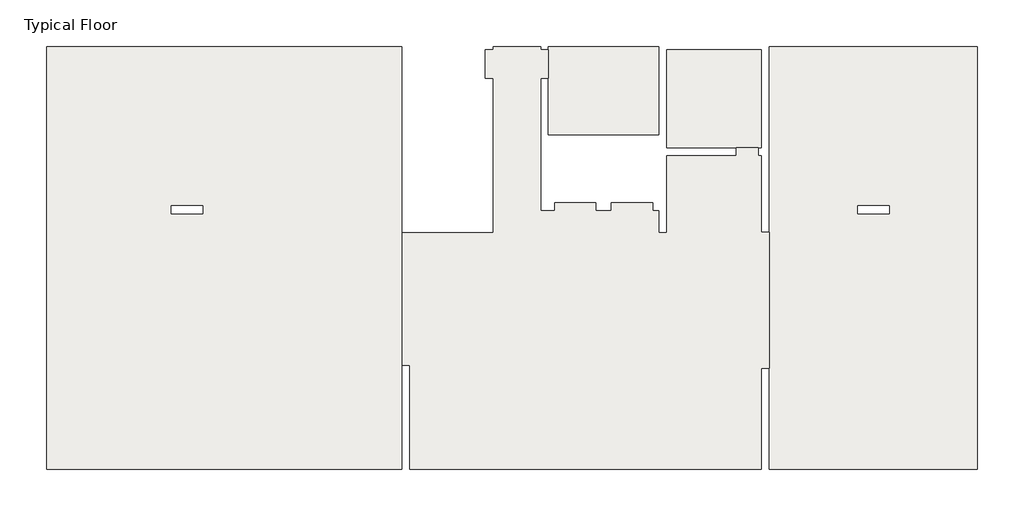
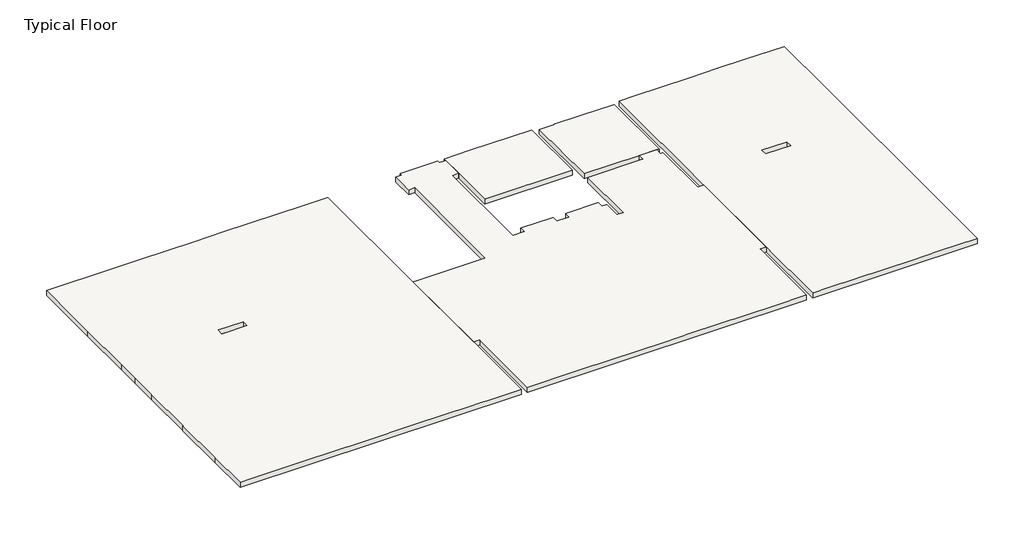
# One storey: 5 slabs.
"""IFC4 building model written with IfcOpenShell, lengths in millimetres."""

from ifc_helpers import new_model, si_unit, origin, place, context, project, spatial, faceted_brep, element, save

model = new_model("IFC4")

# Units and contexts
model_context = context("Model", 3, world=origin())
ifc_project = project(units=[si_unit("LENGTHUNIT", "METRE", prefix="MILLI")], contexts=[model_context])

# Site, building, storey
site = spatial("IfcSite", under=ifc_project)
building = spatial("IfcBuilding", under=site)
storey = spatial("IfcBuildingStorey", under=building, Name="Typical Floor", Elevation=3500.0)

# Slabs
placement = place(None, origin())
element("IfcSlab", 1, ObjectType="21", at=placement, inside=storey, context=model_context, shape_type="Brep", body=[
    faceted_brep([(67.1459865, 8440.4665211, 3290.0), (67.1459865, 2544.8683269, 3290.0), (67.1459865, -1658.0097769, 3290.0), (67.1459865, -4954.849506, 3290.0), (-11182.5718465, -4954.849506, 3290.0), (-11182.5718465, -3207.1068424, 3290.0), (-11187.5718465, -3207.1068424, 3290.0), (-11187.5718465, -1006.2039078, 3290.0), (-11182.5718465, -1006.2039078, 3290.0), (-11182.5718465, 1194.6990267, 3290.0), (-11187.5718465, 1194.6990267, 3290.0), (-11187.5718465, 2290.9179883, 3290.0), (-11182.5718465, 2290.9179883, 3290.0), (-11182.5718465, 3268.626792, 3290.0), (-11187.5718465, 3268.626792, 3290.0), (-11187.5718465, 5592.2723901, 3290.0), (-11182.5718465, 5592.2723901, 3290.0), (-11182.5718465, 8440.4665211, 3290.0), (-6230.8224108, 3391.6516226, 3290.0), (-7230.8224108, 3391.6516226, 3290.0), (-7230.8224108, 3141.6516226, 3290.0), (-6230.8224108, 3141.6516226, 3290.0), (67.1459865, -4954.849506, 3500.0), (67.1459865, -1658.0097769, 3500.0), (67.1459865, 2544.8683269, 3500.0), (67.1459865, 8440.4665211, 3500.0), (-830.1452099, 8440.4665211, 3500.0), (-1930.5966772, 8440.4665211, 3500.0), (-4131.4996117, 8440.4665211, 3500.0), (-5232.8540135, 8440.4665211, 3500.0), (-7432.8540135, 8440.4665211, 3500.0), (-8529.0729751, 8440.4665211, 3500.0), (-11182.5718465, 8440.4665211, 3500.0), (-11182.5718465, 5592.2723901, 3500.0), (-11187.5718465, 5592.2723901, 3500.0), (-11187.5718465, 3268.626792, 3500.0), (-11182.5718465, 3268.626792, 3500.0), (-11182.5718465, 2290.9179883, 3500.0), (-11187.5718465, 2290.9179883, 3500.0), (-11187.5718465, 1194.6990267, 3500.0), (-11182.5718465, 1194.6990267, 3500.0), (-11182.5718465, -1006.2039078, 3500.0), (-11187.5718465, -1006.2039078, 3500.0), (-11187.5718465, -3207.1068424, 3500.0), (-11182.5718465, -3207.1068424, 3500.0), (-11182.5718465, -4954.849506, 3500.0), (-8529.0729751, -4954.849506, 3500.0), (-7432.8540135, -4954.849506, 3500.0), (-6332.4025462, -4954.849506, 3500.0), (-4131.4996117, -4954.849506, 3500.0), (-1930.5966772, -4954.849506, 3500.0), (-830.1452099, -4954.849506, 3500.0), (-7230.8224108, 3391.6516226, 3500.0), (-6230.8224108, 3391.6516226, 3500.0), (-6230.8224108, 3141.6516226, 3500.0), (-7230.8224108, 3141.6516226, 3500.0)], [[[0, 1, 2, 3, 4, 5, 6, 7, 8, 9, 10, 11, 12, 13, 14, 15, 16, 17], [18, 19, 20, 21]], [[22, 23, 24, 25, 26, 27, 28, 29, 30, 31, 32, 33, 34, 35, 36, 37, 38, 39, 40, 41, 42, 43, 44, 45, 46, 47, 48, 49, 50, 51], [52, 53, 54, 55]], [[3, 2, 1, 0, 25, 24, 23, 22]], [[3, 22, 51, 50, 49, 48, 47, 46, 45, 4]], [[6, 43, 42, 7]], [[10, 39, 38, 11]], [[14, 35, 34, 15]], [[25, 0, 17, 32, 31, 30, 29, 28, 27, 26]], [[18, 53, 52, 19]], [[53, 18, 21, 54]], [[54, 21, 20, 55]], [[55, 20, 19, 52]], [[44, 5, 4, 45]], [[5, 44, 43, 6]], [[8, 41, 40, 9]], [[9, 40, 39, 10]], [[41, 8, 7, 42]], [[12, 37, 36, 13]], [[13, 36, 35, 14]], [[37, 12, 11, 38]], [[16, 33, 32, 17]], [[33, 16, 15, 34]]]),
])
element("IfcSlab", 2, ObjectType="21", at=placement, inside=storey, context=model_context, shape_type="Brep", body=[
    faceted_brep([(2966.4123522, 2544.8683269, 3290.0), (2966.4123522, 7441.8773563, 3290.0), (2716.4123522, 7441.8773563, 3290.0), (2716.4123522, 8343.4010583, 3290.0), (2966.4123522, 8343.4010583, 3290.0), (2966.4123522, 8440.4665211, 3290.0), (4468.6696885, 8440.4665211, 3290.0), (4468.6696885, 8343.4010583, 3290.0), (4718.6696885, 8343.4010583, 3290.0), (4718.6696885, 7441.8773563, 3290.0), (4468.9518556, 7441.8773563, 3290.0), (4468.9518556, 3493.2317581, 3290.0), (4468.9518556, 3243.2317581, 3290.0), (4926.0624651, 3243.2317581, 3290.0), (4926.0624651, 3493.2317581, 3290.0), (6216.9766863, 3493.2317581, 3290.0), (6216.9766863, 3243.2317581, 3290.0), (6716.4123522, 3243.2317581, 3290.0), (6716.4123522, 3493.2317581, 3290.0), (8020.0240903, 3493.2317581, 3290.0), (8020.0240903, 3243.2317581, 3290.0), (8218.6696885, 3243.2317581, 3290.0), (8218.6696885, 2544.8683269, 3290.0), (8468.6696885, 2544.8683269, 3290.0), (8468.6696885, 4990.9744217, 3290.0), (10669.5726231, 4990.9744217, 3290.0), (10669.5726231, 5240.9744217, 3290.0), (11372.1685599, 5240.9744217, 3290.0), (11372.1685599, 4991.2565888, 3290.0), (11469.2340226, 4991.2565888, 3290.0), (11469.2340226, 2566.0308552, 3290.0), (11719.2340226, 2566.0308552, 3290.0), (11719.2340226, -1755.3574067, 3290.0), (11469.2340226, -1755.3574067, 3290.0), (11469.2340226, -4954.849506, 3290.0), (317.1459865, -4954.849506, 3290.0), (317.1459865, -1658.0097769, 3290.0), (67.1459865, -1658.0097769, 3290.0), (67.1459865, 2544.8683269, 3290.0), (317.1459865, 2544.8683269, 3290.0), (2716.4123522, 2544.8683269, 3290.0), (2966.4123522, 7441.8773563, 3500.0), (2966.4123522, 2544.8683269, 3500.0), (2716.4123522, 2544.8683269, 3500.0), (317.1459865, 2544.8683269, 3500.0), (67.1459865, 2544.8683269, 3500.0), (67.1459865, -1658.0097769, 3500.0), (317.1459865, -1658.0097769, 3500.0), (317.1459865, -4954.849506, 3500.0), (2466.9766863, -4954.849506, 3500.0), (5768.3310881, -4954.849506, 3500.0), (6868.7825554, -4954.849506, 3500.0), (9069.6854899, -4954.849506, 3500.0), (10165.9044515, -4954.849506, 3500.0), (11469.2340226, -4954.849506, 3500.0), (11469.2340226, -1755.3574067, 3500.0), (11719.2340226, -1755.3574067, 3500.0), (11719.2340226, 2566.0308552, 3500.0), (11469.2340226, 2566.0308552, 3500.0), (11469.2340226, 4991.2565888, 3500.0), (11372.1685599, 4991.2565888, 3500.0), (11372.1685599, 5240.9744217, 3500.0), (10669.5726231, 5240.9744217, 3500.0), (10669.5726231, 4990.9744217, 3500.0), (8468.6696885, 4990.9744217, 3500.0), (8468.6696885, 2544.8683269, 3500.0), (8218.6696885, 2544.8683269, 3500.0), (8218.6696885, 3243.2317581, 3500.0), (8020.0240903, 3243.2317581, 3500.0), (8020.0240903, 3493.2317581, 3500.0), (6716.4123522, 3493.2317581, 3500.0), (6716.4123522, 3243.2317581, 3500.0), (6216.9766863, 3243.2317581, 3500.0), (6216.9766863, 3493.2317581, 3500.0), (4926.0624651, 3493.2317581, 3500.0), (4926.0624651, 3243.2317581, 3500.0), (4468.9518556, 3243.2317581, 3500.0), (4468.9518556, 3493.2317581, 3500.0), (4468.9518556, 7441.8773563, 3500.0), (4718.6696885, 7441.8773563, 3500.0), (4718.6696885, 8343.4010583, 3500.0), (4468.6696885, 8343.4010583, 3500.0), (4468.6696885, 8440.4665211, 3500.0), (2966.4123522, 8440.4665211, 3500.0), (2966.4123522, 8343.4010583, 3500.0), (2716.4123522, 8343.4010583, 3500.0), (2716.4123522, 7441.8773563, 3500.0)], [[[0, 1, 2, 3, 4, 5, 6, 7, 8, 9, 10, 11, 12, 13, 14, 15, 16, 17, 18, 19, 20, 21, 22, 23, 24, 25, 26, 27, 28, 29, 30, 31, 32, 33, 34, 35, 36, 37, 38, 39, 40]], [[41, 42, 43, 44, 45, 46, 47, 48, 49, 50, 51, 52, 53, 54, 55, 56, 57, 58, 59, 60, 61, 62, 63, 64, 65, 66, 67, 68, 69, 70, 71, 72, 73, 74, 75, 76, 77, 78, 79, 80, 81, 82, 83, 84, 85, 86]], [[1, 0, 42, 41]], [[6, 5, 83, 82]], [[10, 78, 77, 76, 12, 11]], [[22, 21, 67, 66]], [[23, 22, 66, 65]], [[24, 23, 65, 64]], [[30, 29, 59, 58]], [[31, 30, 58, 57]], [[32, 31, 57, 56]], [[33, 32, 56, 55]], [[34, 33, 55, 54]], [[35, 34, 54, 53, 52, 51, 50, 49, 48]], [[36, 35, 48, 47]], [[37, 36, 47, 46]], [[38, 37, 46, 45]], [[38, 45, 44, 43, 42, 0, 40, 39]], [[2, 1, 41, 86]], [[3, 2, 86, 85]], [[4, 3, 85, 84]], [[5, 4, 84, 83]], [[7, 6, 82, 81]], [[8, 7, 81, 80]], [[9, 8, 80, 79]], [[10, 9, 79, 78]], [[13, 12, 76, 75]], [[14, 13, 75, 74]], [[15, 14, 74, 73]], [[16, 15, 73, 72]], [[17, 16, 72, 71]], [[18, 17, 71, 70]], [[19, 18, 70, 69]], [[20, 19, 69, 68]], [[21, 20, 68, 67]], [[25, 24, 64, 63]], [[26, 25, 63, 62]], [[27, 26, 62, 61]], [[28, 27, 61, 60]], [[29, 28, 60, 59]]]),
])
element("IfcSlab", 3, ObjectType="21", at=placement, inside=storey, context=model_context, shape_type="Brep", body=[
    faceted_brep([(18317.4281535, -4954.849506, 3290.0), (11719.2340226, -4954.849506, 3290.0), (11719.2340226, -1755.3574067, 3290.0), (11719.2340226, 2566.0308552, 3290.0), (11719.2340226, 8440.7486881, 3290.0), (14567.7103206, 8440.7486881, 3290.0), (14567.7103206, 8440.4665211, 3290.0), (15668.1617879, 8440.4665211, 3290.0), (15668.1617879, 8440.7486881, 3290.0), (16768.6132551, 8440.7486881, 3290.0), (16768.6132551, 8440.4665211, 3290.0), (18317.4281535, 8440.4665211, 3290.0), (15515.7915847, 3391.6516226, 3290.0), (14515.7915847, 3391.6516226, 3290.0), (14515.7915847, 3141.6516226, 3290.0), (15515.7915847, 3141.6516226, 3290.0), (11719.2340226, -4954.849506, 3500.0), (12366.8073861, -4954.849506, 3500.0), (13467.2588533, -4954.849506, 3500.0), (15668.1617879, -4954.849506, 3500.0), (16768.6132551, -4954.849506, 3500.0), (18317.4281535, -4954.849506, 3500.0), (18317.4281535, -3207.1068424, 3500.0), (18317.4281535, -2106.6553751, 3500.0), (18317.4281535, 1194.6990267, 3500.0), (18317.4281535, 2290.9179883, 3500.0), (18317.4281535, 4491.8209229, 3500.0), (18317.4281535, 5600.7374014, 3500.0), (18317.4281535, 8440.4665211, 3500.0), (16768.6132551, 8440.4665211, 3500.0), (16768.6132551, 8440.7486881, 3500.0), (15668.1617879, 8440.7486881, 3500.0), (15668.1617879, 8440.4665211, 3500.0), (14567.7103206, 8440.4665211, 3500.0), (14567.7103206, 8440.7486881, 3500.0), (12366.8073861, 8440.7486881, 3500.0), (11719.2340226, 8440.7486881, 3500.0), (11719.2340226, 2566.0308552, 3500.0), (11719.2340226, -1755.3574067, 3500.0), (14515.7915847, 3391.6516226, 3500.0), (15515.7915847, 3391.6516226, 3500.0), (15515.7915847, 3141.6516226, 3500.0), (14515.7915847, 3141.6516226, 3500.0)], [[[0, 1, 2, 3, 4, 5, 6, 7, 8, 9, 10, 11], [12, 13, 14, 15]], [[16, 17, 18, 19, 20, 21, 22, 23, 24, 25, 26, 27, 28, 29, 30, 31, 32, 33, 34, 35, 36, 37, 38], [39, 40, 41, 42]], [[21, 0, 11, 28, 27, 26, 25, 24, 23, 22]], [[1, 0, 21, 20, 19, 18, 17, 16]], [[4, 3, 2, 1, 16, 38, 37, 36]], [[8, 31, 30, 9]], [[4, 36, 35, 34, 5]], [[12, 40, 39, 13]], [[40, 12, 15, 41]], [[41, 15, 14, 42]], [[42, 14, 13, 39]], [[6, 33, 32, 7]], [[7, 32, 31, 8]], [[33, 6, 5, 34]], [[10, 29, 28, 11]], [[29, 10, 9, 30]]]),
])
element("IfcSlab", 4, ObjectType="21", at=placement, inside=storey, context=model_context, shape_type="Brep", body=[
    faceted_brep([(8218.6696885, 5643.0624579, 3290.0), (4718.9518556, 5643.0624579, 3290.0), (4718.9518556, 7441.8773563, 3290.0), (4718.6696885, 7441.8773563, 3290.0), (4718.6696885, 8343.4010583, 3290.0), (4718.6696885, 8445.4665211, 3290.0), (5768.3310881, 8445.4665211, 3290.0), (5768.3310881, 8440.4665211, 3290.0), (8218.6696885, 8440.4665211, 3290.0), (4718.9518556, 5643.0624579, 3500.0), (8218.6696885, 5643.0624579, 3500.0), (8218.6696885, 8440.4665211, 3500.0), (5768.3310881, 8440.4665211, 3500.0), (5768.3310881, 8445.4665211, 3500.0), (4718.6696885, 8445.4665211, 3500.0), (4718.6696885, 8343.4010583, 3500.0), (4718.6696885, 7441.8773563, 3500.0), (4718.9518556, 7441.8773563, 3500.0)], [[[0, 1, 2, 3, 4, 5, 6, 7, 8]], [[9, 10, 11, 12, 13, 14, 15, 16, 17]], [[14, 5, 4, 3, 16, 15]], [[5, 14, 13, 6]], [[10, 0, 8, 11]], [[0, 10, 9, 1]], [[17, 2, 1, 9]], [[2, 17, 16, 3]], [[7, 12, 11, 8]], [[12, 7, 6, 13]]]),
])
element("IfcSlab", 5, ObjectType="21", at=placement, inside=storey, context=model_context, shape_type="Brep", body=[
    faceted_brep([(11469.2340226, 5241.2565888, 3290.0), (11372.1685599, 5241.2565888, 3290.0), (11372.1685599, 5240.9744217, 3290.0), (10669.5726231, 5240.9744217, 3290.0), (8468.6696885, 5240.9744217, 3290.0), (8468.6696885, 8340.4665211, 3290.0), (9069.6854899, 8340.4665211, 3290.0), (9069.6854899, 8345.4665211, 3290.0), (10165.9044515, 8345.4665211, 3290.0), (10165.9044515, 8340.4665211, 3290.0), (11469.2340226, 8340.4665211, 3290.0), (11372.1685599, 5241.2565888, 3500.0), (11469.2340226, 5241.2565888, 3500.0), (11469.2340226, 8340.4665211, 3500.0), (10165.9044515, 8340.4665211, 3500.0), (10165.9044515, 8345.4665211, 3500.0), (9069.6854899, 8345.4665211, 3500.0), (9069.6854899, 8340.4665211, 3500.0), (8468.6696885, 8340.4665211, 3500.0), (8468.6696885, 5240.9744217, 3500.0), (10669.5726231, 5240.9744217, 3500.0), (11372.1685599, 5240.9744217, 3500.0)], [[[0, 1, 2, 3, 4, 5, 6, 7, 8, 9, 10]], [[11, 12, 13, 14, 15, 16, 17, 18, 19, 20, 21]], [[12, 0, 10, 13]], [[19, 4, 3, 2, 21, 20]], [[4, 19, 18, 5]], [[7, 16, 15, 8]], [[11, 1, 0, 12]], [[1, 11, 21, 2]], [[17, 6, 5, 18]], [[6, 17, 16, 7]], [[9, 14, 13, 10]], [[14, 9, 8, 15]]]),
])

save(model, "model.ifc")

# Revit data of these elements
# Type "21"
#   Function = 0
#   Layers, outside or top first: 21 cm "Concrete" (function 1)
# Element 1 (IfcSlab, "21")
#   Mark = "S1"
#   SOFiSTiK_AMG_Comments = ""
#   Height Offset From Level = 0 cm
#   built-in parameter 1001954 = 1
#   SOFiSTiK_AMG_Scheduled = yes
#   SOFiSTiK_AMG_Adjusted = yes
#   Phase Created = New Construction
#   Materials on its faces: "Concrete"
# Element 2 (IfcSlab, "21")
#   Mark = "S2"
#   SOFiSTiK_AMG_Comments = ""
#   Height Offset From Level = 0 cm
#   built-in parameter 1001954 = 1
#   SOFiSTiK_AMG_Scheduled = yes
#   SOFiSTiK_AMG_Adjusted = yes
#   Phase Created = New Construction
#   Materials on its faces: "Concrete"
# Element 3 (IfcSlab, "21")
#   Mark = "S3"
#   SOFiSTiK_AMG_Comments = ""
#   Height Offset From Level = 0 cm
#   built-in parameter 1001954 = 1
#   SOFiSTiK_AMG_Scheduled = yes
#   SOFiSTiK_AMG_Adjusted = yes
#   Phase Created = New Construction
#   Materials on its faces: "Concrete"
# Element 4 (IfcSlab, "21")
#   Mark = "S4"
#   SOFiSTiK_AMG_Comments = ""
#   built-in parameter 1001955 = 3.14159 (stored number, unit not read)
#   Height Offset From Level = 0 cm
#   built-in parameter 1001954 = 1
#   SOFiSTiK_AMG_Scheduled = yes
#   SOFiSTiK_AMG_Adjusted = yes
#   Phase Created = New Construction
#   Materials on its faces: "Concrete"
# Element 5 (IfcSlab, "21")
#   Mark = "S5"
#   SOFiSTiK_AMG_Comments = ""
#   Height Offset From Level = 0 cm
#   built-in parameter 1001954 = 1
#   SOFiSTiK_AMG_Scheduled = yes
#   SOFiSTiK_AMG_Adjusted = yes
#   Phase Created = New Construction
#   Materials on its faces: "Concrete"
# Materials
#   "Concrete": class "Concrete", colour RGB 192 192 192, transparency 0, Keynote = "01000", Description = "Cast-in-place concrete", Cost = 0
